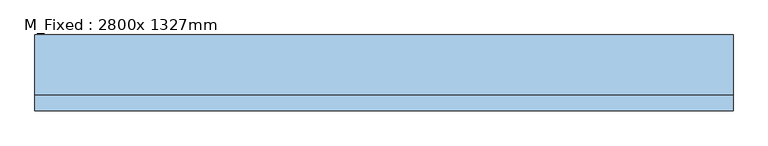
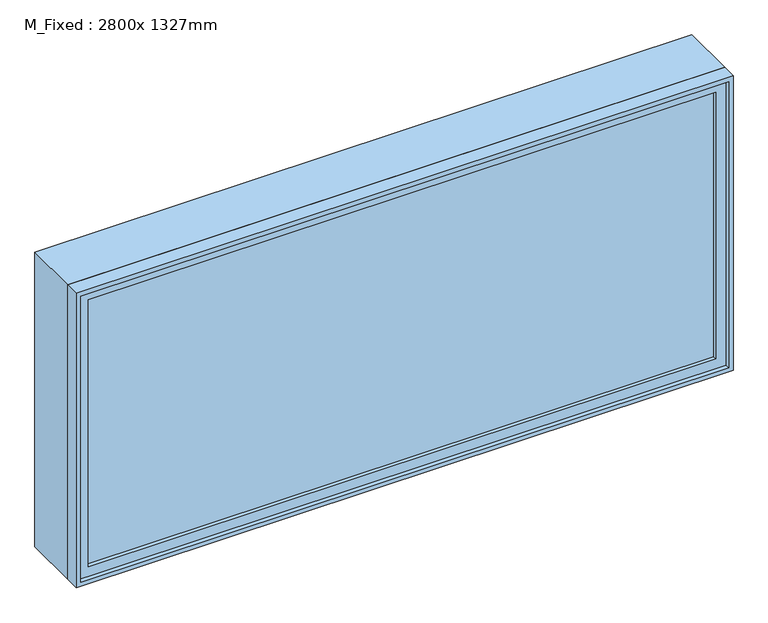
"""IFC4 building model written with IfcOpenShell, lengths in millimetres: window geometry, M_Fixed : 2800x 1327mm."""

from ifc_helpers import new_model, si_unit, frame, origin, place, context, project, spatial, polyline, outline, extrude, source, transform, mapped, element, save


def m_fixed_2800x_1327mm_95955449(model_context):
    return source(origin(), model_context, "Body", "SweptSolid", [
        extrude(outline(polyline([(-1337.0, -130.4), (-1337.0, -118.4), (1337.0, -118.4), (1337.0, -130.4), (-1337.0, -130.4)])), frame((0.0, 0.0, 978.0), z_axis=(0.0, 0.0, 1.0), x_axis=(1.0, 0.0, 0.0)), (0.0, 0.0, 1.0), 1201.2),
        extrude(outline(polyline([(2223.2, -1381.0), (934.0, -1381.0), (934.0, 1381.0), (2223.2, 1381.0), (2223.2, -1381.0)]), holes=[polyline([(2179.2, -1337.0), (2179.2, 1337.0), (978.0, 1337.0), (978.0, -1337.0), (2179.2, -1337.0)])]), frame((0.0, -146.4, 0.0), z_axis=(0.0, 1.0, 0.0), x_axis=(0.0, 0.0, 1.0)), (0.0, 0.0, 1.0), 44.0),
        extrude(outline(polyline([(2242.2, -1400.0), (915.0, -1400.0), (915.0, 1400.0), (2242.2, 1400.0), (2242.2, -1400.0)]), holes=[polyline([(2223.2, -1381.0), (2223.2, 1381.0), (934.0, 1381.0), (934.0, -1381.0), (2223.2, -1381.0)])]), frame((0.0, -165.4, 0.0), z_axis=(0.0, 1.0, 0.0), x_axis=(0.0, 0.0, 1.0)), (0.0, 0.0, 1.0), 63.0),
        extrude(outline(polyline([(2242.2, -1400.0), (915.0, -1400.0), (915.0, 1400.0), (2242.2, 1400.0), (2242.2, -1400.0)]), holes=[polyline([(2210.2, -1368.0), (2210.2, 1368.0), (947.0, 1368.0), (947.0, -1368.0), (2210.2, -1368.0)])]), frame((0.0, -102.4, 0.0), z_axis=(0.0, 1.0, 0.0), x_axis=(0.0, 0.0, 1.0)), (0.0, 0.0, 1.0), 241.8),
    ])


if __name__ == "__main__":
    model = new_model("IFC4")
    model_context = context("Model", 3, world=origin())
    ifc_project = project(units=[si_unit("LENGTHUNIT", "METRE", prefix="MILLI")], contexts=[model_context])
    site = spatial("IfcSite", under=ifc_project)
    building = spatial("IfcBuilding", under=site)
    placement = place(None, origin())
    m_fixed_2800x_1327mm_shape = m_fixed_2800x_1327mm_95955449(model_context)
    element("IfcWindow", 1, ObjectType="M_Fixed : 2800x 1327mm", at=placement, inside=building, context=model_context, shape_type="MappedRepresentation", body=[
        mapped(m_fixed_2800x_1327mm_shape, transform((0.0, 0.0, 0.0), x_axis=(1.0, 0.0, 0.0), y_axis=(0.0, 1.0, 0.0), z_axis=(0.0, 0.0, 1.0))),
    ])
    save(model, "model.ifc")

# Revit data of these elements
# Type "M_Fixed : 2800x 1327mm"
#   Type Mark = "46"
#   Height = 1327.2 mm
#   Default Sill Height = 915 mm
#   Width = 2800 mm
#   Window Inset = 19 mm
#   Frame Exterior Material = Sash
#   Frame Interior Material = Sash
#   Glass Pane Material = Glass
#   Sash = Sash
#   Wall Closure = (empty or 0)
# Element 1 (IfcWindow, "M_Fixed : 2800x 1327mm")
#   Materials on its faces: "Sash", "Glass"
# Materials
#   "Sash": class "Wood", colour RGB 136 99 55, transparency 0
#   "Glass": class "Glass", colour RGB 0 128 192, transparency 0.9, Description = "Soda Lime Glass", Cost = 0
